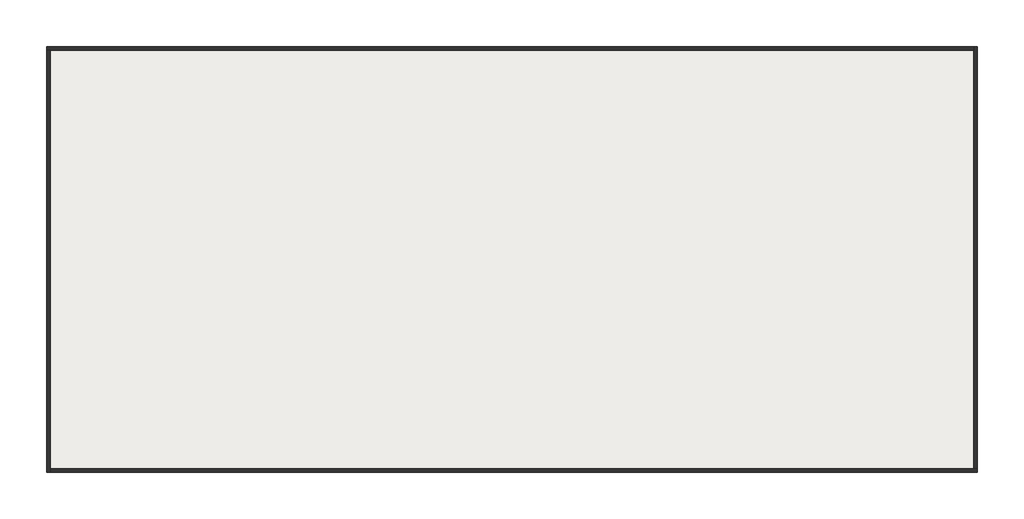
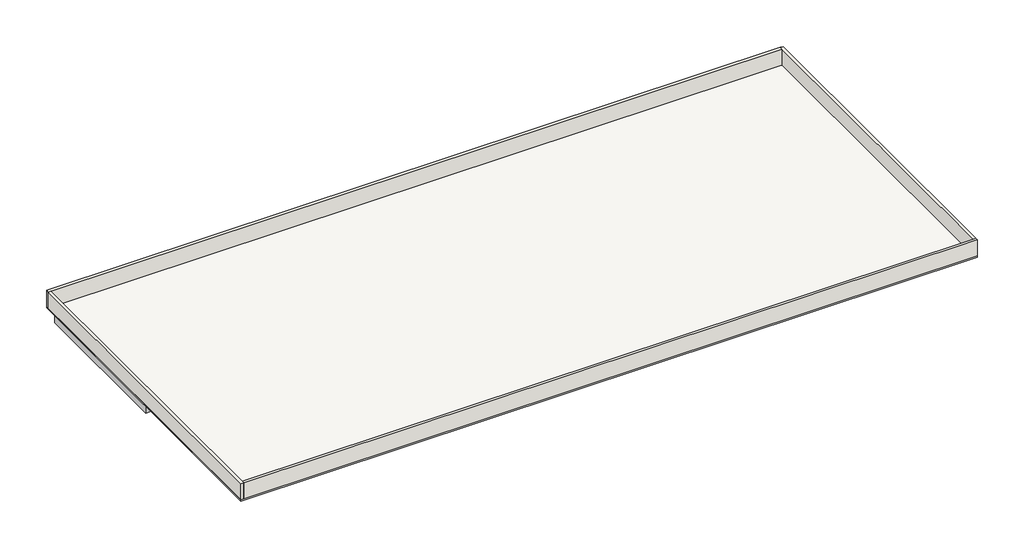
# One storey: 9 beams, 4 walls, 1 roof.
"""IFC4 building model written with IfcOpenShell, lengths in millimetres."""

from ifc_helpers import new_model, si_unit, frame, origin, place, context, project, spatial, polyline, outline, extrude, faceted_brep, element, save

model = new_model("IFC4")

# Units and contexts
model_context = context("Model", 3, world=origin())
ifc_project = project(units=[si_unit("LENGTHUNIT", "METRE", prefix="MILLI")], contexts=[model_context])

# Site, building, storey
site = spatial("IfcSite", under=ifc_project)
building = spatial("IfcBuilding", under=site)
storey = spatial("IfcBuildingStorey", under=building, Name="TOC", Elevation=7650.0)

# Beams
placement = place(None, origin())
element("IfcBeam", 1, ObjectType="RC Beam_Rectangular : H_SB_ACB_B400xH900", at=placement, inside=storey, context=model_context, shape_type="SweptSolid", body=[
    extrude(outline(polyline([(12616.5208589, 6750.0), (12616.5208589, 7500.0), (12303.8208589, 7500.0), (12303.8208589, 7549.0), (24429.2208589, 7549.0), (24429.2208589, 7500.0), (24116.5208589, 7500.0), (24116.5208589, 6750.0), (12616.5208589, 6750.0)])), frame((-275.3, 0.0, 0.0), z_axis=(1.0, 0.0, 0.0), x_axis=(0.0, 1.0, 0.0)), (0.0, 0.0, 1.0), 400.0),
])
element("IfcBeam", 2, ObjectType="RC Beam_Rectangular : H_SB_ACB_B400xH900", at=placement, inside=storey, context=model_context, shape_type="SweptSolid", body=[
    extrude(outline(polyline([(12616.5208589, 6750.0), (12616.5208589, 7500.0), (12303.8208589, 7500.0), (12303.8208589, 7549.0), (24429.2208589, 7549.0), (24429.2208589, 7500.0), (24116.5208589, 7500.0), (24116.5208589, 6750.0), (12616.5208589, 6750.0)])), frame((5724.7, 0.0, 0.0), z_axis=(1.0, 0.0, 0.0), x_axis=(0.0, 1.0, 0.0)), (0.0, 0.0, 1.0), 400.0),
])
element("IfcBeam", 3, ObjectType="RC Beam_Rectangular : H_SB_ACB_B400xH900", at=placement, inside=storey, context=model_context, shape_type="SweptSolid", body=[
    extrude(outline(polyline([(12616.5208589, 6750.0), (12616.5208589, 7500.0), (12303.8208589, 7500.0), (12303.8208589, 7549.0), (24429.2208589, 7549.0), (24429.2208589, 7500.0), (24116.5208589, 7500.0), (24116.5208589, 6750.0), (12616.5208589, 6750.0)])), frame((11724.7, 0.0, 0.0), z_axis=(1.0, 0.0, 0.0), x_axis=(0.0, 1.0, 0.0)), (0.0, 0.0, 1.0), 400.0),
])
element("IfcBeam", 4, ObjectType="RC Beam_Rectangular : H_SB_ACB_B400xH900", at=placement, inside=storey, context=model_context, shape_type="SweptSolid", body=[
    extrude(outline(polyline([(12616.5208589, 6750.0), (12616.5208589, 7500.0), (12303.8208589, 7500.0), (12303.8208589, 7549.0), (24429.2208589, 7549.0), (24429.2208589, 7500.0), (24116.5208589, 7500.0), (24116.5208589, 6750.0), (12616.5208589, 6750.0)])), frame((17724.7, 0.0, 0.0), z_axis=(1.0, 0.0, 0.0), x_axis=(0.0, 1.0, 0.0)), (0.0, 0.0, 1.0), 400.0),
])
element("IfcBeam", 5, ObjectType="RC Beam_Rectangular : H_SB_ACB_B400xH900", at=placement, inside=storey, context=model_context, shape_type="SweptSolid", body=[
    extrude(outline(polyline([(12516.5208589, 7500.0), (12303.8208589, 7500.0), (12303.8208589, 7549.0), (24429.2208589, 7549.0), (24429.2208589, 7500.0), (24116.5208589, 7500.0), (24116.5208589, 6750.0), (12516.5208589, 6750.0), (12516.5208589, 7500.0)])), frame((25924.7, 0.0, 0.0), z_axis=(1.0, 0.0, 0.0), x_axis=(0.0, 1.0, 0.0)), (0.0, 0.0, 1.0), 400.0),
])
element("IfcBeam", 6, ObjectType="RC Beam_Rectangular : H_SB_ACB_B400xH900", at=placement, inside=storey, context=model_context, shape_type="SweptSolid", body=[
    extrude(outline(polyline([(12516.5208589, 7500.0), (12303.8208589, 7500.0), (12303.8208589, 7549.0), (24429.2208589, 7549.0), (24429.2208589, 7500.0), (24116.5208589, 7500.0), (24116.5208589, 6750.0), (12516.5208589, 6750.0), (12516.5208589, 7500.0)])), frame((31724.7, 0.0, 0.0), z_axis=(1.0, 0.0, 0.0), x_axis=(0.0, 1.0, 0.0)), (0.0, 0.0, 1.0), 400.0),
])
element("IfcBeam", 7, ObjectType="RC Beam_Rectangular : H_SB_ACB_B400xH900", at=placement, inside=storey, context=model_context, shape_type="SweptSolid", body=[
    extrude(outline(polyline([(12516.5208589, 7500.0), (12303.8208589, 7500.0), (12303.8208589, 7549.0), (24429.2208589, 7549.0), (24429.2208589, 7500.0), (24116.5208589, 7500.0), (24116.5208589, 6750.0), (12516.5208589, 6750.0), (12516.5208589, 7500.0)])), frame((38724.7, 0.0, 0.0), z_axis=(1.0, 0.0, 0.0), x_axis=(0.0, 1.0, 0.0)), (0.0, 0.0, 1.0), 400.0),
])
element("IfcBeam", 8, ObjectType="RC Beam_Rectangular : H_SB_ACB_B400xH900", at=placement, inside=storey, context=model_context, shape_type="SweptSolid", body=[
    extrude(outline(polyline([(12516.5208589, 7500.0), (12303.8208589, 7500.0), (12303.8208589, 7549.0), (24429.2208589, 7549.0), (24429.2208589, 7500.0), (24116.5208589, 7500.0), (24116.5208589, 6750.0), (12516.5208589, 6750.0), (12516.5208589, 7500.0)])), frame((45724.7, 0.0, 0.0), z_axis=(1.0, 0.0, 0.0), x_axis=(0.0, 1.0, 0.0)), (0.0, 0.0, 1.0), 400.0),
])
element("IfcBeam", 9, ObjectType="RC Beam_Rectangular : H_SB_ACB_B400xH900", at=placement, inside=storey, context=model_context, shape_type="SweptSolid", body=[
    extrude(outline(polyline([(24116.5208589, 7500.0), (24116.5208589, 6750.0), (12516.5208589, 6750.0), (12516.5208589, 7500.0), (12303.8208589, 7500.0), (12303.8208589, 7549.0), (24429.2208589, 7549.0), (24429.2208589, 7500.0), (24116.5208589, 7500.0)])), frame((52724.7, 0.0, 0.0), z_axis=(1.0, 0.0, 0.0), x_axis=(0.0, 1.0, 0.0)), (0.0, 0.0, 1.0), 400.0),
])

# Roof
element("IfcRoof", 10, ObjectType="H_RF_AMF_RC Roof Finish_WP_Insulation_Protection", at=placement, inside=storey, context=model_context, shape_type="SweptSolid", body=[
    extrude(outline(polyline([(53324.7, 24816.5208589), (53324.7, 216.5208589), (-475.3, 216.5208589), (-475.3, 24816.5208589), (53324.7, 24816.5208589)])), frame((0.0, 0.0, 7549.0), z_axis=(0.0, 0.0, 1.0), x_axis=(1.0, 0.0, 0.0)), (0.0, 0.0, 1.0), 101.0),
])

# Walls
element("IfcWall", 11, ObjectType="H_WA_AMW_RC Wall_T200 (No Finish)", at=placement, inside=storey, context=model_context, shape_type="Brep", body=[
    faceted_brep([(-475.3, 24616.5208589, 7650.0), (-275.3, 24616.5208589, 7650.0), (53124.7, 24616.5208589, 7650.0), (53124.7, 24616.5208589, 8900.0), (-275.3, 24616.5208589, 8900.0), (-475.3, 24616.5208589, 8900.0), (-475.3, 24816.5208589, 7650.0), (-475.3, 24816.5208589, 8900.0), (53124.7, 24816.5208589, 8900.0), (53124.7, 24816.5208589, 7650.0)], [[[0, 1, 2, 3, 4, 5]], [[6, 7, 8, 9]], [[2, 1, 0, 6, 9]], [[5, 4, 3, 8, 7]], [[0, 5, 7, 6]], [[3, 2, 9, 8]]]),
])
element("IfcWall", 12, ObjectType="H_WA_AMW_RC Wall_T200 (No Finish)", at=placement, inside=storey, context=model_context, shape_type="Brep", body=[
    faceted_brep([(-275.3, 216.5208589, 7650.0), (-275.3, 416.5208589, 7650.0), (-275.3, 24616.5208589, 7650.0), (-275.3, 24616.5208589, 8900.0), (-275.3, 416.5208589, 8900.0), (-275.3, 216.5208589, 8900.0), (-475.3, 216.5208589, 7650.0), (-475.3, 216.5208589, 8900.0), (-475.3, 24616.5208589, 8900.0), (-475.3, 24616.5208589, 7650.0)], [[[0, 1, 2, 3, 4, 5]], [[6, 7, 8, 9]], [[2, 1, 0, 6, 9]], [[5, 4, 3, 8, 7]], [[0, 5, 7, 6]], [[3, 2, 9, 8]]]),
])
element("IfcWall", 13, ObjectType="H_WA_AMW_RC Wall_T200 (No Finish)", at=placement, inside=storey, context=model_context, shape_type="Brep", body=[
    faceted_brep([(53324.7, 416.5208589, 7650.0), (53124.7, 416.5208589, 7650.0), (-275.3, 416.5208589, 7650.0), (-275.3, 416.5208589, 8900.0), (53124.7, 416.5208589, 8900.0), (53324.7, 416.5208589, 8900.0), (53324.7, 216.5208589, 7650.0), (53324.7, 216.5208589, 8900.0), (-275.3, 216.5208589, 8900.0), (-275.3, 216.5208589, 7650.0)], [[[0, 1, 2, 3, 4, 5]], [[6, 7, 8, 9]], [[2, 1, 0, 6, 9]], [[5, 4, 3, 8, 7]], [[0, 5, 7, 6]], [[3, 2, 9, 8]]]),
])
element("IfcWall", 14, ObjectType="H_WA_AMW_RC Wall_T200 (No Finish)", at=placement, inside=storey, context=model_context, shape_type="Brep", body=[
    faceted_brep([(53124.7, 24816.5208589, 7650.0), (53124.7, 24616.5208589, 7650.0), (53124.7, 416.5208589, 7650.0), (53124.7, 416.5208589, 8900.0), (53124.7, 24616.5208589, 8900.0), (53124.7, 24816.5208589, 8900.0), (53324.7, 24816.5208589, 7650.0), (53324.7, 24816.5208589, 8900.0), (53324.7, 416.5208589, 8900.0), (53324.7, 416.5208589, 7650.0)], [[[0, 1, 2, 3, 4, 5]], [[6, 7, 8, 9]], [[2, 1, 0, 6, 9]], [[5, 4, 3, 8, 7]], [[0, 5, 7, 6]], [[3, 2, 9, 8]]]),
])

save(model, "model.ifc")

# Revit data of these elements
# Type "RC Beam_Rectangular : H_SB_ACB_B400xH900"
#   중앙부 하부근 = ""
#   중앙부 상부근 = ""
#   중앙부 보조근 = ""
#   중앙부 늑근 = ""
#   외단부 하부근 = ""
#   외단부 상부근 = ""
#   외단부 보조근 = ""
#   외단부 늑근 = ""
#   부호 = "TG3"
#   내단부 하부근 = ""
#   내단부 상부근 = ""
#   내단부 보조근 = ""
#   내단부 늑근 = ""
#   ALL 하부근 = "3-D20"
#   ALL 상부근 = "3-D20"
#   ALL 보조근 = ""
#   ALL 늑근 = "2-D10 @120"
#   Width = 400.000 mm
#   Height = 900.000 mm
#   Length [instance default] = 1524.000 mm
#   b = 400.000 mm
#   h = 900.000 mm
#   hec_material3 [instance default] = none
#   hec_material2 [instance default] = none
#   hec_material1 [instance default] = none
#   Structural Material [instance default] = none
#   Assembly Code = ""
# Type "H_RF_AMF_RC Roof Finish_WP_Insulation_Protection"
#   Layers, outside or top first: 50.000 mm no material (function 4); 0.000 mm no material (function 100); 50.000 mm no material (function 3); 1.000 mm no material (function 2)
# Type "H_WA_AMW_RC Wall_T200 (No Finish)"
#   Type Comments = ""
#   Layers, outside or top first: 0.000 mm no material (function 100); 0.000 mm no material (function 100); 200.000 mm no material (function 1); 0.000 mm no material (function 100); 0.000 mm no material (function 100); 0.000 mm no material (function 100)
# Elements 1, 2, 3, 4, 5, 6, 7, 8, 9 (IfcBeam, "RC Beam_Rectangular : H_SB_ACB_B400xH900")
#   hec_material3 = none
#   hec_material2 = none
#   hec_material1 = none
#   Structural Material = none
#   Phase Created = New Construction
# Element 10 (IfcRoof, "H_RF_AMF_RC Roof Finish_WP_Insulation_Protection")
#   built-in parameter 1001705 = 25.0984 (stored number, unit not read)
#   built-in parameter 1001701 = -0.331365 (stored number, unit not read)
#   built-in parameter 1001710 = 33615
#   Phase Created = New Construction
#   Materials on its faces: "Default Roof"
# Elements 11, 12, 13, 14 (IfcWall, "H_WA_AMW_RC Wall_T200 (No Finish)")
#   Top Offset = 0.000 mm
#   Base Offset = 0.000 mm
#   wall height = 1250.000 mm
#   Phase Created = New Construction
#   Base Constraint = TOC
#   Top Constraint = TOP
#   Materials on its faces: "Default Wall"
# Materials
#   "Default Roof": class "Miscellaneous", colour RGB 80 80 80, transparency 0
#   "Default Wall": class "Miscellaneous", colour RGB 80 80 80, transparency 0
